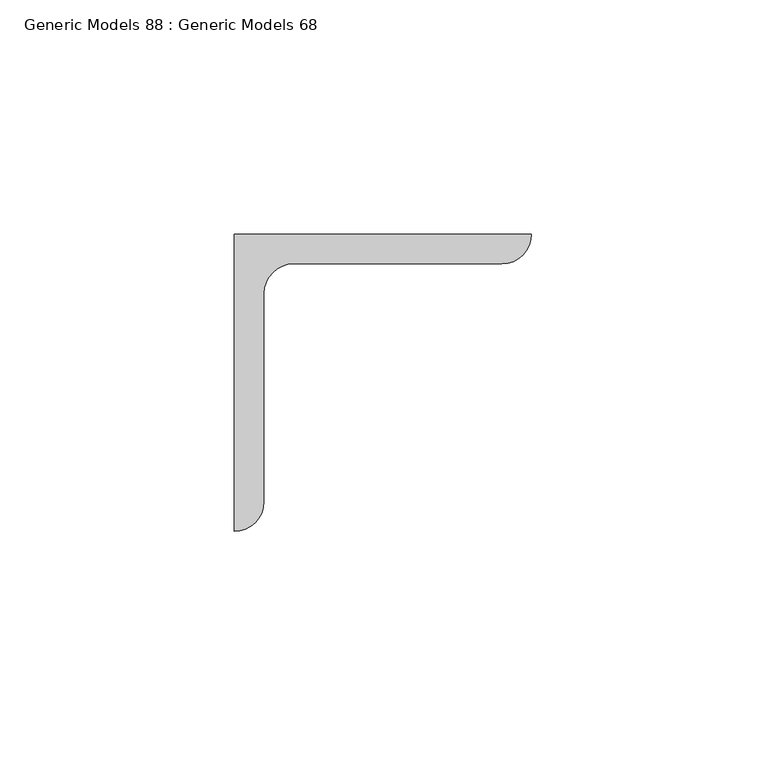
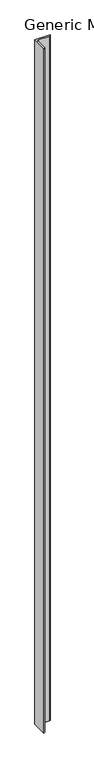
"""IFC4 building model written with IfcOpenShell, lengths in millimetres: proxy geometry, Generic Models 88 : Generic Models 68."""

from ifc_helpers import new_model, si_unit, point, frame, frame_2d, origin, place, context, project, spatial, polyline, circle_curve, trimmed, segment, composite_curve, outline, extrude, source, transform, mapped, element, save


def generic_models_88_generic_models_68_aea504db(model_context):
    return source(origin(), model_context, "Body", "SweptSolid", [
        extrude(outline(composite_curve([segment(polyline([(20530.4116945, 20934.4264581), (20593.9116945, 20934.4264581)]), True, "CONTINUOUS"), segment(trimmed(circle_curve(frame_2d((20587.5616945, 20934.4264581)), 6.35), [point((20593.9116945, 20934.4264581))], [point((20587.5616945, 20928.0764581))], False, "CARTESIAN"), True, "CONTINUOUS"), segment(polyline([(20587.5616945, 20928.0764581), (20543.1116945, 20928.0764581)]), True, "CONTINUOUS"), segment(trimmed(circle_curve(frame_2d((20543.1116945, 20921.7264581)), 6.35), [point((20543.1116945, 20928.0764581))], [point((20536.7616945, 20921.7264581))], True, "CARTESIAN"), True, "CONTINUOUS"), segment(polyline([(20536.7616945, 20921.7264581), (20536.7616945, 20877.2764581)]), True, "CONTINUOUS"), segment(trimmed(circle_curve(frame_2d((20530.4116945, 20877.2764581)), 6.35), [point((20536.7616945, 20877.2764581))], [point((20530.4116945, 20870.9264581))], False, "CARTESIAN"), True, "CONTINUOUS"), segment(polyline([(20530.4116945, 20870.9264581), (20530.4116945, 20934.4264581)]), True, "CONTINUOUS")], self_intersect=False)), frame((0.0, 0.0, 264380.6186948), z_axis=(0.0, 0.0, 1.0), x_axis=(1.0, 0.0, 0.0)), (0.0, 0.0, 1.0), 3006.09),
    ])


if __name__ == "__main__":
    model = new_model("IFC4")
    model_context = context("Model", 3, world=origin())
    ifc_project = project(units=[si_unit("LENGTHUNIT", "METRE", prefix="MILLI")], contexts=[model_context])
    site = spatial("IfcSite", under=ifc_project)
    building = spatial("IfcBuilding", under=site)
    placement = place(None, origin())
    generic_models_88_generic_models_68_shape = generic_models_88_generic_models_68_aea504db(model_context)
    element("IfcBuildingElementProxy", 1, Name="Generic Models 88 : Generic Models 68", ObjectType="Generic Models 88 : Generic Models 68", at=placement, inside=building, context=model_context, shape_type="MappedRepresentation", body=[
        mapped(generic_models_88_generic_models_68_shape, transform((0.0, 0.0, 0.0), x_axis=(1.0, 0.0, 0.0), y_axis=(0.0, 1.0, 0.0), z_axis=(0.0, 0.0, 1.0))),
    ])
    save(model, "model.ifc")

# Revit data of these elements
# Element 1 (IfcBuildingElementProxy, "Generic Models 88 : Generic Models 68")
#   Materials on its faces: "MAIN FENCE POST: (2) BACK/BACK GALVANIZED ANGLES (2) L2 1/2 X 2 1/2 X 1/4\") ANCHORED TO 8\"W X 42\" DEEP CONCRETE FOOTING(1)"
# Materials
#   "MAIN FENCE POST: (2) BACK/BACK GALVANIZED ANGLES (2) L2 1/2 X 2 1/2 X 1/4\") ANCHORED TO 8\"W X 42\" DEEP CONCRETE FOOTING(1)": class "Unassigned", colour RGB 211 211 211, transparency 0, Cost = 0
